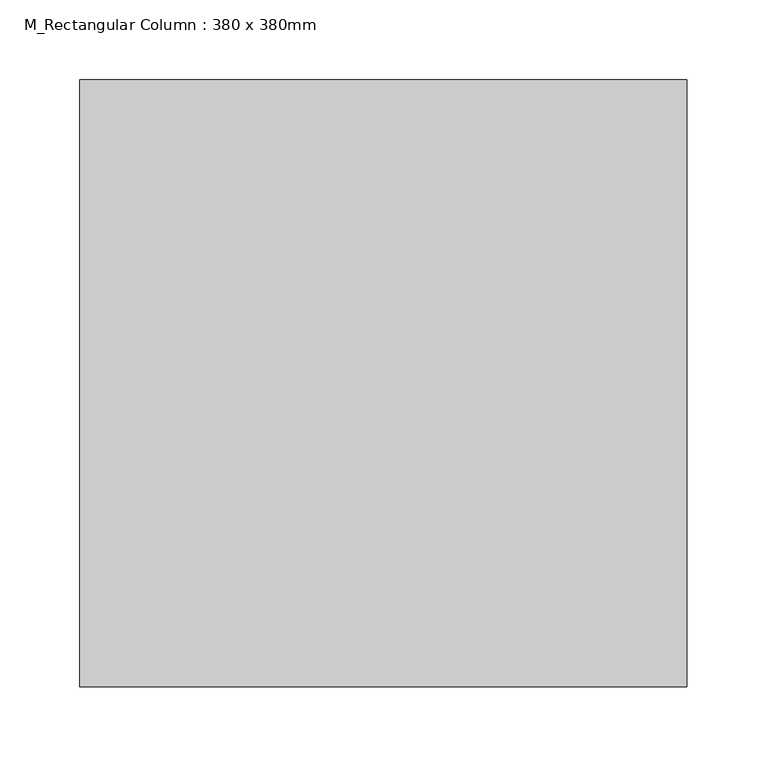
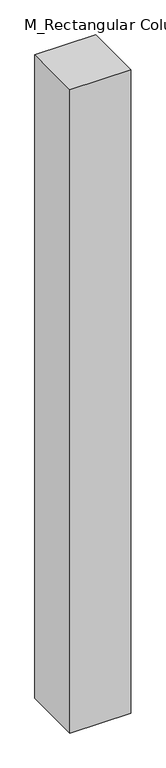
"""IFC4 building model written with IfcOpenShell, lengths in millimetres: column geometry, M_Rectangular Column : 380 x 380mm."""

import ifcopenshell
import ifcopenshell.guid

model = None  # the IFC model being written
_history = None  # IfcOwnerHistory: only IFC2X3 demands one
_inside = {}  # id of a spatial element -> (the spatial element, [elements in it])
_under = {}  # id of a project, library or spatial element -> (it, [spatial elements below it])
_declared = {}  # id of a project -> (the project, [libraries it declares])
_typed = {}  # id of a type object -> (the type object, [elements of that type])
_made_of = {}  # id of a material, layer set ... -> (it, [elements and type objects made of it])


def new_model(schema):
    """Start an empty IFC model of exactly this schema.

    Asked for "IFC4X3", IfcOpenShell would pick the latest addendum, in which some entities
    have other attributes; the version numbers below select the first issue.
    IFC2X3 requires an IfcOwnerHistory on every rooted entity: one is made here for all.
    """
    global model, _history
    if schema == "IFC4X3":
        model = ifcopenshell.file(schema_version=(4, 3, 0, 0))
    else:
        model = ifcopenshell.file(schema=schema)
    _inside.clear()
    _under.clear()
    _declared.clear()
    _typed.clear()
    _made_of.clear()
    _history = None
    if model.schema == "IFC2X3":
        org = make("IfcOrganization", Name="unknown")
        user = make(
            "IfcPersonAndOrganization",
            ThePerson=make("IfcPerson", FamilyName="unknown"),
            TheOrganization=org,
        )
        app = make(
            "IfcApplication",
            ApplicationDeveloper=org,
            Version="unknown",
            ApplicationFullName="unknown",
            ApplicationIdentifier="unknown",
        )
        _history = make(
            "IfcOwnerHistory",
            OwningUser=user,
            OwningApplication=app,
            ChangeAction="ADDED",
            CreationDate=0,
        )
    return model


def make(cls, **values):
    """One entity of the class cls with the attributes given. An attribute that is None is left unset."""
    return model.create_entity(
        cls, **{name: value for name, value in values.items() if value is not None}
    )


def rooted(cls, **values):
    """An entity with a GlobalId (a new one), such as an element, a storey or a relation."""
    return make(cls, GlobalId=ifcopenshell.guid.new(), OwnerHistory=_history, **values)


def si_unit(unit_type, name, prefix=None):
    """IfcSIUnit, for example si_unit("LENGTHUNIT", "METRE", prefix="MILLI")."""
    return make("IfcSIUnit", UnitType=unit_type, Prefix=prefix, Name=name)


def assignment(units):
    """IfcUnitAssignment: the units of a project."""
    return None if units is None else make("IfcUnitAssignment", Units=units)


def point(xyz):
    """IfcCartesianPoint."""
    return None if xyz is None else make("IfcCartesianPoint", Coordinates=xyz)


def direction(xyz):
    """IfcDirection."""
    return None if xyz is None else make("IfcDirection", DirectionRatios=xyz)


def frame(location, z_axis=None, x_axis=None):
    """IfcAxis2Placement3D, a coordinate frame: its origin and axes. An axis left out is left unset."""
    return make(
        "IfcAxis2Placement3D",
        Location=point(location),
        Axis=direction(z_axis),
        RefDirection=direction(x_axis),
    )


def origin():
    """The frame at (0, 0, 0) with its axes left unset."""
    return frame((0.0, 0.0, 0.0))


def place(relative_to, where):
    """IfcLocalPlacement: puts the frame where relative to a parent placement (None: the world)."""
    return make(
        "IfcLocalPlacement", PlacementRelTo=relative_to, RelativePlacement=where
    )


def context(
    kind, dimensions, precision=None, world=None, true_north=None, identifier=None
):
    """IfcGeometricRepresentationContext, for example the 3D "Model" context."""
    return make(
        "IfcGeometricRepresentationContext",
        ContextIdentifier=identifier,
        ContextType=kind,
        CoordinateSpaceDimension=dimensions,
        Precision=precision,
        WorldCoordinateSystem=world,
        TrueNorth=true_north,
    )


def project(units=None, contexts=None):
    """IfcProject with its units and contexts."""
    return rooted(
        "IfcProject",
        Name="project",
        RepresentationContexts=contexts,
        UnitsInContext=assignment(units),
    )


def spatial(cls, under=None, at=None, **own):
    """A site, building, storey or space (cls), placed at a placement, below another one or the project."""
    s = rooted(cls, ObjectPlacement=at, **own)
    if under is not None:
        _under.setdefault(under.id(), (under, []))[1].append(s)
    return s


def polyline(points):
    """IfcPolyline through the points."""
    return make("IfcPolyline", Points=[point(p) for p in points])


def outline(outer, holes=None, kind="AREA"):
    """IfcArbitraryClosedProfileDef: a profile drawn as a closed curve; with holes, ...WithVoids."""
    if holes is None:
        return make("IfcArbitraryClosedProfileDef", ProfileType=kind, OuterCurve=outer)
    return make(
        "IfcArbitraryProfileDefWithVoids",
        ProfileType=kind,
        OuterCurve=outer,
        InnerCurves=holes,
    )


def extrude(swept, where, along, depth):
    """IfcExtrudedAreaSolid: the profile swept, set in the frame where, extruded along a direction by depth."""
    return make(
        "IfcExtrudedAreaSolid",
        SweptArea=swept,
        Position=where,
        ExtrudedDirection=direction(along),
        Depth=depth,
    )


def shape(context_of_items, identifier, shape_type, items):
    """IfcShapeRepresentation: the items that make up one representation, for example the "Body"."""
    return make(
        "IfcShapeRepresentation",
        ContextOfItems=context_of_items,
        RepresentationIdentifier=identifier,
        RepresentationType=shape_type,
        Items=items,
    )


def source(mapping_origin, context_of_items, identifier, shape_type, items):
    """IfcRepresentationMap: a shape defined once, which mapped items show again and again."""
    return make(
        "IfcRepresentationMap",
        MappingOrigin=mapping_origin,
        MappedRepresentation=shape(context_of_items, identifier, shape_type, items),
    )


def transform(
    local_origin,
    x_axis=None,
    y_axis=None,
    z_axis=None,
    scale=None,
    scale2=None,
    scale3=None,
    uniform=True,
):
    """IfcCartesianTransformationOperator3D, or its non-uniform kind. x_axis, y_axis, z_axis: its Axis1, 2, 3."""
    if uniform:
        return make(
            "IfcCartesianTransformationOperator3D",
            Axis1=direction(x_axis),
            Axis2=direction(y_axis),
            LocalOrigin=point(local_origin),
            Scale=scale,
            Axis3=direction(z_axis),
        )
    return make(
        "IfcCartesianTransformationOperator3DnonUniform",
        Axis1=direction(x_axis),
        Axis2=direction(y_axis),
        LocalOrigin=point(local_origin),
        Scale=scale,
        Axis3=direction(z_axis),
        Scale2=scale2,
        Scale3=scale3,
    )


def mapped(mapping_source, mapping_target):
    """IfcMappedItem: shows the shape of a source again, moved by a transform."""
    return make(
        "IfcMappedItem", MappingSource=mapping_source, MappingTarget=mapping_target
    )


def made_of(thing, what):
    """Note that an element or type object is made of a material, layer set ...; save() writes the relation."""
    if what is not None:
        _made_of.setdefault(what.id(), (what, []))[1].append(thing)
    return thing


def element(
    cls,
    number,
    at=None,
    inside=None,
    cuts=None,
    type_object=None,
    material=None,
    context=None,
    identifier="Body",
    shape_type=None,
    held_by="IfcProductDefinitionShape",
    body=None,
    shapes=None,
    **own,
):
    """One element of the class cls, such as IfcWall. Its Tag is "e" and its number.

    at: its placement. inside: the storey or other place that contains it. cuts: it is an
    opening in that element (IfcRelVoidsElement). A single representation is given by context,
    identifier, shape_type and body (its items); several are given by shapes. held_by: the class
    of the entity that holds the representations. save() writes the other relations.
    """
    e = rooted(cls, Tag="e%d" % number, ObjectPlacement=at, **own)
    if body is not None:
        shapes = [shape(context, identifier, shape_type, body)]
    if shapes is not None:
        e.Representation = make(held_by, Representations=shapes)
    if inside is not None:
        _inside.setdefault(inside.id(), (inside, []))[1].append(e)
    if cuts is not None:
        rooted(
            "IfcRelVoidsElement", RelatingBuildingElement=cuts, RelatedOpeningElement=e
        )
    if type_object is not None:
        _typed.setdefault(type_object.id(), (type_object, []))[1].append(e)
    return made_of(e, material)


def aggregate(whole, parts):
    """IfcRelAggregates: a whole, such as a stair, and the parts it consists of."""
    return rooted("IfcRelAggregates", RelatingObject=whole, RelatedObjects=parts)


def save(model, path):
    """Write the relations noted so far, then the file.

    IfcRelAggregates (storeys below a building ...), IfcRelContainedInSpatialStructure (elements
    in a storey), IfcRelDefinesByType, IfcRelAssociatesMaterial and IfcRelDeclares: one each for
    every whole, place, type object, material and project.
    """
    for whole, parts in _under.values():
        aggregate(whole, parts)
    for where, things in _inside.values():
        rooted(
            "IfcRelContainedInSpatialStructure",
            RelatedElements=things,
            RelatingStructure=where,
        )
    for kind, things in _typed.values():
        rooted("IfcRelDefinesByType", RelatedObjects=things, RelatingType=kind)
    for what, things in _made_of.values():
        rooted("IfcRelAssociatesMaterial", RelatedObjects=things, RelatingMaterial=what)
    for by, libraries in _declared.values():
        rooted("IfcRelDeclares", RelatingContext=by, RelatedDefinitions=libraries)
    model.write(path)


def m_rectangular_column_380_x_380mm_f7aa0fc7(model_context):
    return source(origin(), model_context, "Body", "SweptSolid", [
        extrude(outline(polyline([(190.0, 190.0), (190.0, -190.0), (-190.0, -190.0), (-190.0, 190.0), (190.0, 190.0)])), frame((0.0, 0.0, 40.0), z_axis=(0.0, 0.0, 1.0), x_axis=(1.0, 0.0, 0.0)), (0.0, 0.0, 1.0), 4260.0),
    ])


if __name__ == "__main__":
    model = new_model("IFC4")
    model_context = context("Model", 3, world=origin())
    ifc_project = project(units=[si_unit("LENGTHUNIT", "METRE", prefix="MILLI")], contexts=[model_context])
    site = spatial("IfcSite", under=ifc_project)
    building = spatial("IfcBuilding", under=site)
    placement = place(None, origin())
    m_rectangular_column_380_x_380mm_shape = m_rectangular_column_380_x_380mm_f7aa0fc7(model_context)
    element("IfcColumn", 1, ObjectType="M_Rectangular Column : 380 x 380mm", at=placement, inside=building, context=model_context, shape_type="MappedRepresentation", body=[
        mapped(m_rectangular_column_380_x_380mm_shape, transform((0.0, 0.0, 0.0), x_axis=(1.0, 0.0, 0.0), y_axis=(0.0, 1.0, 0.0), z_axis=(0.0, 0.0, 1.0))),
    ])
    save(model, "model.ifc")

# Revit data of these elements
# Type "M_Rectangular Column : 380 x 380mm"
#   Depth = 38.0 cm
#   Offset Base = 0.0 cm
#   Offset Top = 0.0 cm
#   Width = 38.0 cm
#   Material = none
